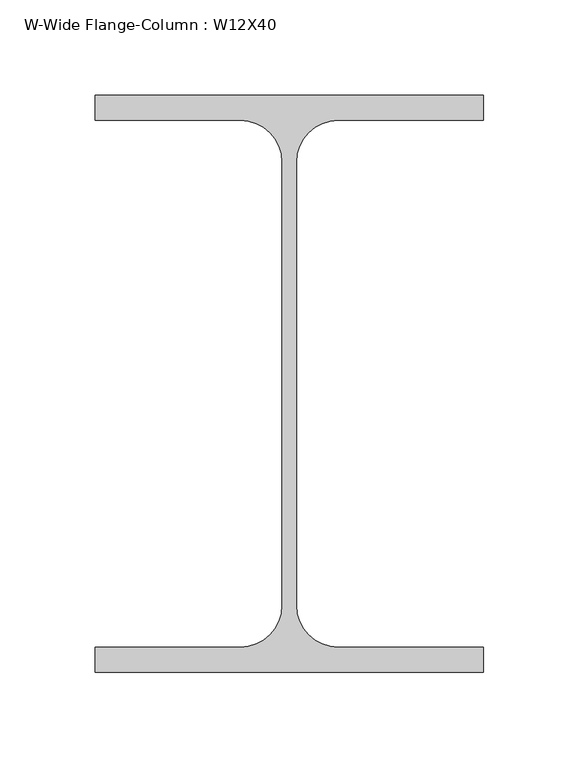
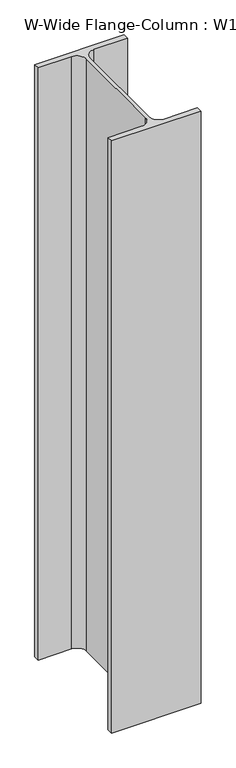
"""IFC4 building model written with IfcOpenShell, lengths in millimetres: column geometry, W-Wide Flange-Column : W12X40."""

from ifc_helpers import new_model, si_unit, point, frame, frame_2d, origin, place, context, project, spatial, polyline, circle_curve, trimmed, segment, composite_curve, outline, extrude, source, transform, mapped, element, save


def w_wide_flange_column_w12x40_442959c1(model_context):
    return source(origin(), model_context, "Body", "SweptSolid", [
        extrude(outline(composite_curve([segment(polyline([(101.727, 151.13), (101.727, 138.049), (25.5905, 138.049)]), True, "CONTINUOUS"), segment(trimmed(circle_curve(frame_2d((25.5905, 116.205)), 21.844), [point((25.5905, 138.049))], [point((3.7465, 116.205))], True, "CARTESIAN"), True, "CONTINUOUS"), segment(polyline([(3.7465, 116.205), (3.7465, -116.205)]), True, "CONTINUOUS"), segment(trimmed(circle_curve(frame_2d((25.5905, -116.205)), 21.844), [point((3.7465, -116.205))], [point((25.5905, -138.049))], True, "CARTESIAN"), True, "CONTINUOUS"), segment(polyline([(25.5905, -138.049), (101.727, -138.049), (101.727, -151.13), (-101.727, -151.13), (-101.727, -138.049), (-25.5905, -138.049)]), True, "CONTINUOUS"), segment(trimmed(circle_curve(frame_2d((-25.5905, -116.205)), 21.844), [point((-25.5905, -138.049))], [point((-3.7465, -116.205))], True, "CARTESIAN"), True, "CONTINUOUS"), segment(polyline([(-3.7465, -116.205), (-3.7465, 116.205)]), True, "CONTINUOUS"), segment(trimmed(circle_curve(frame_2d((-25.5905, 116.205)), 21.844), [point((-3.7465, 116.205))], [point((-25.5905, 138.049))], True, "CARTESIAN"), True, "CONTINUOUS"), segment(polyline([(-25.5905, 138.049), (-101.727, 138.049), (-101.727, 151.13), (101.727, 151.13)]), True, "CONTINUOUS")], self_intersect=False)), frame((0.0, 0.0, 23317.2), z_axis=(0.0, 0.0, 1.0), x_axis=(1.0, 0.0, 0.0)), (0.0, 0.0, 1.0), 1422.4),
    ])


if __name__ == "__main__":
    model = new_model("IFC4")
    model_context = context("Model", 3, world=origin())
    ifc_project = project(units=[si_unit("LENGTHUNIT", "METRE", prefix="MILLI")], contexts=[model_context])
    site = spatial("IfcSite", under=ifc_project)
    building = spatial("IfcBuilding", under=site)
    placement = place(None, origin())
    w_wide_flange_column_w12x40_shape = w_wide_flange_column_w12x40_442959c1(model_context)
    element("IfcColumn", 1, ObjectType="W-Wide Flange-Column : W12X40", at=placement, inside=building, context=model_context, shape_type="MappedRepresentation", body=[
        mapped(w_wide_flange_column_w12x40_shape, transform((0.0, 0.0, 0.0), x_axis=(1.0, 0.0, 0.0), y_axis=(0.0, 1.0, 0.0), z_axis=(0.0, 0.0, 1.0))),
    ])
    save(model, "model.ifc")

# Revit data of these elements
# Type "W-Wide Flange-Column : W12X40"
#   Assembly Code = "B10"
#   W = 40
#   bf = 0' - 8.01"
#   d = 0' - 11.9"
#   k = 0' - 1 3/8"
#   kr = 0' - 0.86"
#   tf = 0' - 0.515"
#   tw = 0' - 0.295"
#   A = 0.08125 SF
#   Structural Material [instance default] = Steel ASTM A992
# Element 1 (IfcColumn, "W-Wide Flange-Column : W12X40")
#   Materials on its faces: "Steel ASTM A992"
# Materials
#   "Steel ASTM A992": class "Metal", colour RGB 199 199 199, transparency 0, Description = "Structural steel 50ksi", Cost = 0
